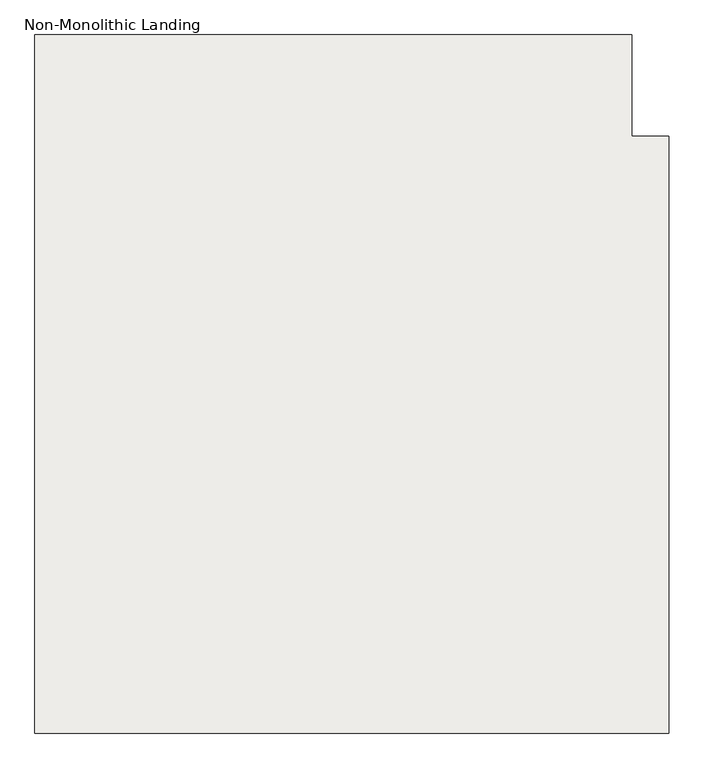
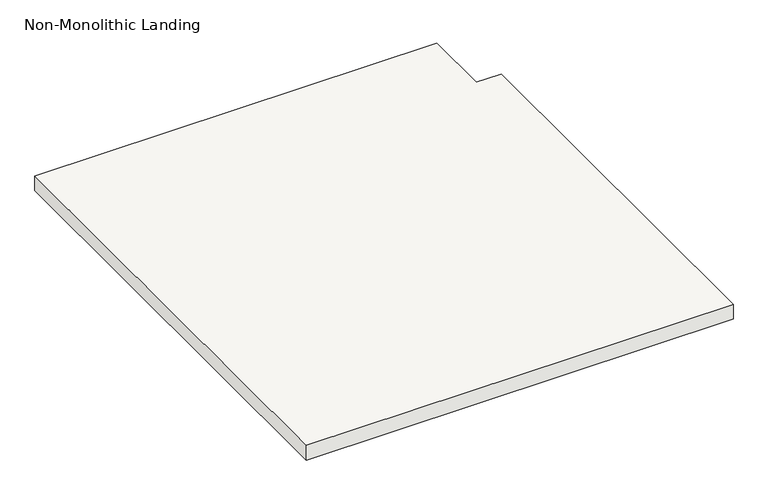
"""IFC4 building model written with IfcOpenShell, lengths in millimetres: slab geometry, Non-Monolithic Landing."""

from ifc_helpers import new_model, si_unit, frame, origin, place, context, project, spatial, polyline, outline, extrude, source, transform, mapped, element, save


def non_monolithic_landing_57dff418(model_context):
    return source(origin(), model_context, "Body", "SweptSolid", [
        extrude(outline(polyline([(-13195.5859635, -3121.1593564), (-14576.101437, -3121.1593564), (-14576.101437, -1600.1378151), (-13276.101437, -1600.1378151), (-13276.101437, -1821.1593564), (-13195.5859635, -1821.1593564), (-13195.5859635, -3121.1593564)])), frame((0.0, 0.0, 1450.0), z_axis=(0.0, 0.0, 1.0), x_axis=(1.0, 0.0, 0.0)), (0.0, 0.0, 1.0), 50.0),
    ])


if __name__ == "__main__":
    model = new_model("IFC4")
    model_context = context("Model", 3, world=origin())
    ifc_project = project(units=[si_unit("LENGTHUNIT", "METRE", prefix="MILLI")], contexts=[model_context])
    site = spatial("IfcSite", under=ifc_project)
    building = spatial("IfcBuilding", under=site)
    placement = place(None, origin())
    non_monolithic_landing_shape = non_monolithic_landing_57dff418(model_context)
    element("IfcSlab", 1, ObjectType="Non-Monolithic Landing", at=placement, inside=building, context=model_context, shape_type="MappedRepresentation", body=[
        mapped(non_monolithic_landing_shape, transform((0.0, 0.0, 0.0), x_axis=(1.0, 0.0, 0.0), y_axis=(0.0, 1.0, 0.0), z_axis=(0.0, 0.0, 1.0))),
    ])
    save(model, "model.ifc")
